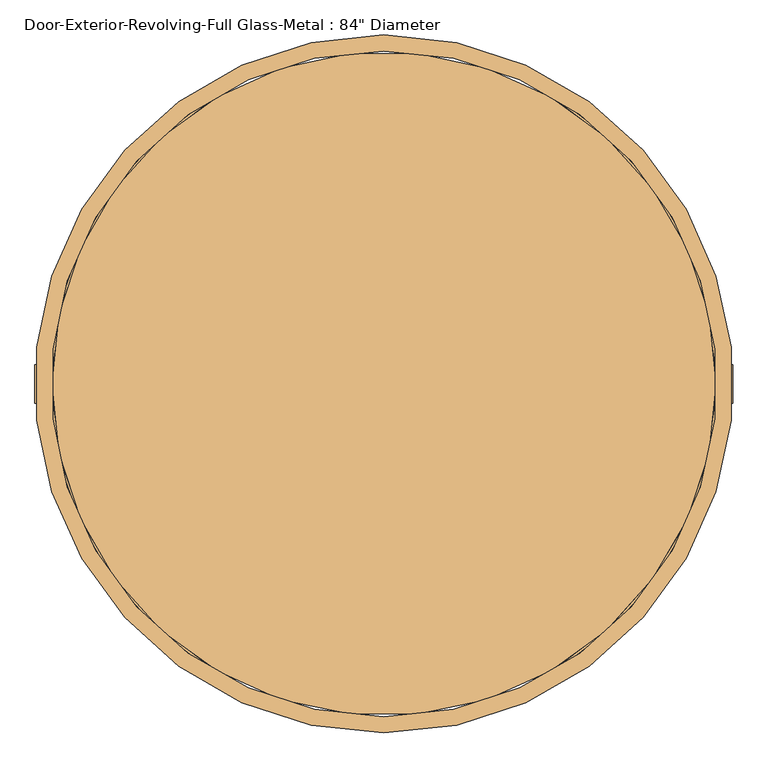
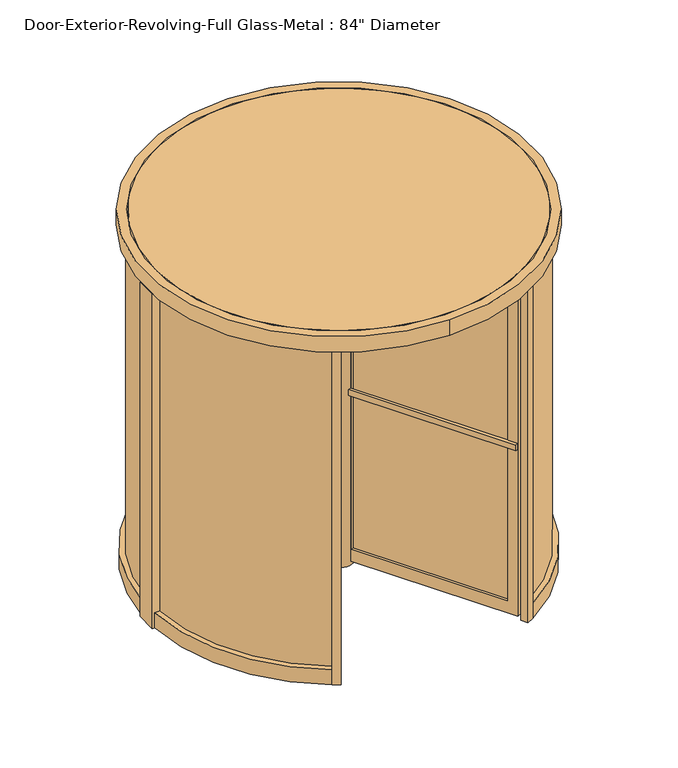
"""IFC4 building model written with IfcOpenShell, lengths in millimetres: door geometry."""

import ifcopenshell
import ifcopenshell.guid

model = None  # the IFC model being written
_history = None  # IfcOwnerHistory: only IFC2X3 demands one
_inside = {}  # id of a spatial element -> (the spatial element, [elements in it])
_under = {}  # id of a project, library or spatial element -> (it, [spatial elements below it])
_declared = {}  # id of a project -> (the project, [libraries it declares])
_typed = {}  # id of a type object -> (the type object, [elements of that type])
_made_of = {}  # id of a material, layer set ... -> (it, [elements and type objects made of it])


def new_model(schema):
    """Start an empty IFC model of exactly this schema.

    Asked for "IFC4X3", IfcOpenShell would pick the latest addendum, in which some entities
    have other attributes; the version numbers below select the first issue.
    IFC2X3 requires an IfcOwnerHistory on every rooted entity: one is made here for all.
    """
    global model, _history
    if schema == "IFC4X3":
        model = ifcopenshell.file(schema_version=(4, 3, 0, 0))
    else:
        model = ifcopenshell.file(schema=schema)
    _inside.clear()
    _under.clear()
    _declared.clear()
    _typed.clear()
    _made_of.clear()
    _history = None
    if model.schema == "IFC2X3":
        org = make("IfcOrganization", Name="unknown")
        user = make(
            "IfcPersonAndOrganization",
            ThePerson=make("IfcPerson", FamilyName="unknown"),
            TheOrganization=org,
        )
        app = make(
            "IfcApplication",
            ApplicationDeveloper=org,
            Version="unknown",
            ApplicationFullName="unknown",
            ApplicationIdentifier="unknown",
        )
        _history = make(
            "IfcOwnerHistory",
            OwningUser=user,
            OwningApplication=app,
            ChangeAction="ADDED",
            CreationDate=0,
        )
    return model


def make(cls, **values):
    """One entity of the class cls with the attributes given. An attribute that is None is left unset."""
    return model.create_entity(
        cls, **{name: value for name, value in values.items() if value is not None}
    )


def rooted(cls, **values):
    """An entity with a GlobalId (a new one), such as an element, a storey or a relation."""
    return make(cls, GlobalId=ifcopenshell.guid.new(), OwnerHistory=_history, **values)


def si_unit(unit_type, name, prefix=None):
    """IfcSIUnit, for example si_unit("LENGTHUNIT", "METRE", prefix="MILLI")."""
    return make("IfcSIUnit", UnitType=unit_type, Prefix=prefix, Name=name)


def assignment(units):
    """IfcUnitAssignment: the units of a project."""
    return None if units is None else make("IfcUnitAssignment", Units=units)


def point(xyz):
    """IfcCartesianPoint."""
    return None if xyz is None else make("IfcCartesianPoint", Coordinates=xyz)


def direction(xyz):
    """IfcDirection."""
    return None if xyz is None else make("IfcDirection", DirectionRatios=xyz)


def frame(location, z_axis=None, x_axis=None):
    """IfcAxis2Placement3D, a coordinate frame: its origin and axes. An axis left out is left unset."""
    return make(
        "IfcAxis2Placement3D",
        Location=point(location),
        Axis=direction(z_axis),
        RefDirection=direction(x_axis),
    )


def frame_2d(location, x_axis=None):
    """IfcAxis2Placement2D, a coordinate frame in the plane: its origin and x axis."""
    return make(
        "IfcAxis2Placement2D", Location=point(location), RefDirection=direction(x_axis)
    )


def origin():
    """The frame at (0, 0, 0) with its axes left unset."""
    return frame((0.0, 0.0, 0.0))


def origin_with_axes():
    """The frame at (0, 0, 0) with the z axis (0, 0, 1) and the x axis (1, 0, 0) written out."""
    return frame((0.0, 0.0, 0.0), z_axis=(0.0, 0.0, 1.0), x_axis=(1.0, 0.0, 0.0))


def origin_2d():
    """The frame at (0, 0) in the plane with its x axis left unset."""
    return frame_2d((0.0, 0.0))


def place(relative_to, where):
    """IfcLocalPlacement: puts the frame where relative to a parent placement (None: the world)."""
    return make(
        "IfcLocalPlacement", PlacementRelTo=relative_to, RelativePlacement=where
    )


def context(
    kind, dimensions, precision=None, world=None, true_north=None, identifier=None
):
    """IfcGeometricRepresentationContext, for example the 3D "Model" context."""
    return make(
        "IfcGeometricRepresentationContext",
        ContextIdentifier=identifier,
        ContextType=kind,
        CoordinateSpaceDimension=dimensions,
        Precision=precision,
        WorldCoordinateSystem=world,
        TrueNorth=true_north,
    )


def project(units=None, contexts=None):
    """IfcProject with its units and contexts."""
    return rooted(
        "IfcProject",
        Name="project",
        RepresentationContexts=contexts,
        UnitsInContext=assignment(units),
    )


def spatial(cls, under=None, at=None, **own):
    """A site, building, storey or space (cls), placed at a placement, below another one or the project."""
    s = rooted(cls, ObjectPlacement=at, **own)
    if under is not None:
        _under.setdefault(under.id(), (under, []))[1].append(s)
    return s


def polyline(points):
    """IfcPolyline through the points."""
    return make("IfcPolyline", Points=[point(p) for p in points])


def circle_curve(where, radius):
    """IfcCircle in the frame where."""
    return make("IfcCircle", Position=where, Radius=radius)


def trimmed(basis, trim1, trim2, sense, master):
    """IfcTrimmedCurve: the piece of a basis curve between two trims."""
    return make(
        "IfcTrimmedCurve",
        BasisCurve=basis,
        Trim1=trim1,
        Trim2=trim2,
        SenseAgreement=sense,
        MasterRepresentation=master,
    )


def segment(curve, same_sense, transition):
    """IfcCompositeCurveSegment."""
    return make(
        "IfcCompositeCurveSegment",
        Transition=transition,
        SameSense=same_sense,
        ParentCurve=curve,
    )


def composite_curve(segments, self_intersect=None):
    """IfcCompositeCurve: segments joined end to end."""
    return make("IfcCompositeCurve", Segments=segments, SelfIntersect=self_intersect)


def outline(outer, holes=None, kind="AREA"):
    """IfcArbitraryClosedProfileDef: a profile drawn as a closed curve; with holes, ...WithVoids."""
    if holes is None:
        return make("IfcArbitraryClosedProfileDef", ProfileType=kind, OuterCurve=outer)
    return make(
        "IfcArbitraryProfileDefWithVoids",
        ProfileType=kind,
        OuterCurve=outer,
        InnerCurves=holes,
    )


def extrude(swept, where, along, depth):
    """IfcExtrudedAreaSolid: the profile swept, set in the frame where, extruded along a direction by depth."""
    return make(
        "IfcExtrudedAreaSolid",
        SweptArea=swept,
        Position=where,
        ExtrudedDirection=direction(along),
        Depth=depth,
    )


def shape(context_of_items, identifier, shape_type, items):
    """IfcShapeRepresentation: the items that make up one representation, for example the "Body"."""
    return make(
        "IfcShapeRepresentation",
        ContextOfItems=context_of_items,
        RepresentationIdentifier=identifier,
        RepresentationType=shape_type,
        Items=items,
    )


def source(mapping_origin, context_of_items, identifier, shape_type, items):
    """IfcRepresentationMap: a shape defined once, which mapped items show again and again."""
    return make(
        "IfcRepresentationMap",
        MappingOrigin=mapping_origin,
        MappedRepresentation=shape(context_of_items, identifier, shape_type, items),
    )


def transform(
    local_origin,
    x_axis=None,
    y_axis=None,
    z_axis=None,
    scale=None,
    scale2=None,
    scale3=None,
    uniform=True,
):
    """IfcCartesianTransformationOperator3D, or its non-uniform kind. x_axis, y_axis, z_axis: its Axis1, 2, 3."""
    if uniform:
        return make(
            "IfcCartesianTransformationOperator3D",
            Axis1=direction(x_axis),
            Axis2=direction(y_axis),
            LocalOrigin=point(local_origin),
            Scale=scale,
            Axis3=direction(z_axis),
        )
    return make(
        "IfcCartesianTransformationOperator3DnonUniform",
        Axis1=direction(x_axis),
        Axis2=direction(y_axis),
        LocalOrigin=point(local_origin),
        Scale=scale,
        Axis3=direction(z_axis),
        Scale2=scale2,
        Scale3=scale3,
    )


def mapped(mapping_source, mapping_target):
    """IfcMappedItem: shows the shape of a source again, moved by a transform."""
    return make(
        "IfcMappedItem", MappingSource=mapping_source, MappingTarget=mapping_target
    )


def made_of(thing, what):
    """Note that an element or type object is made of a material, layer set ...; save() writes the relation."""
    if what is not None:
        _made_of.setdefault(what.id(), (what, []))[1].append(thing)
    return thing


def element(
    cls,
    number,
    at=None,
    inside=None,
    cuts=None,
    type_object=None,
    material=None,
    context=None,
    identifier="Body",
    shape_type=None,
    held_by="IfcProductDefinitionShape",
    body=None,
    shapes=None,
    **own,
):
    """One element of the class cls, such as IfcWall. Its Tag is "e" and its number.

    at: its placement. inside: the storey or other place that contains it. cuts: it is an
    opening in that element (IfcRelVoidsElement). A single representation is given by context,
    identifier, shape_type and body (its items); several are given by shapes. held_by: the class
    of the entity that holds the representations. save() writes the other relations.
    """
    e = rooted(cls, Tag="e%d" % number, ObjectPlacement=at, **own)
    if body is not None:
        shapes = [shape(context, identifier, shape_type, body)]
    if shapes is not None:
        e.Representation = make(held_by, Representations=shapes)
    if inside is not None:
        _inside.setdefault(inside.id(), (inside, []))[1].append(e)
    if cuts is not None:
        rooted(
            "IfcRelVoidsElement", RelatingBuildingElement=cuts, RelatedOpeningElement=e
        )
    if type_object is not None:
        _typed.setdefault(type_object.id(), (type_object, []))[1].append(e)
    return made_of(e, material)


def aggregate(whole, parts):
    """IfcRelAggregates: a whole, such as a stair, and the parts it consists of."""
    return rooted("IfcRelAggregates", RelatingObject=whole, RelatedObjects=parts)


def save(model, path):
    """Write the relations noted so far, then the file.

    IfcRelAggregates (storeys below a building ...), IfcRelContainedInSpatialStructure (elements
    in a storey), IfcRelDefinesByType, IfcRelAssociatesMaterial and IfcRelDeclares: one each for
    every whole, place, type object, material and project.
    """
    for whole, parts in _under.values():
        aggregate(whole, parts)
    for where, things in _inside.values():
        rooted(
            "IfcRelContainedInSpatialStructure",
            RelatedElements=things,
            RelatingStructure=where,
        )
    for kind, things in _typed.values():
        rooted("IfcRelDefinesByType", RelatedObjects=things, RelatingType=kind)
    for what, things in _made_of.values():
        rooted("IfcRelAssociatesMaterial", RelatedObjects=things, RelatingMaterial=what)
    for by, libraries in _declared.values():
        rooted("IfcRelDeclares", RelatingContext=by, RelatedDefinitions=libraries)
    model.write(path)


def plane_surface(at):
    """IfcPlane: the flat surface through the origin of the frame at, square to its z axis."""
    return make("IfcPlane", Position=at)


def revolved_surface(curve, axis_point, axis_direction):
    """IfcSurfaceOfRevolution: the curve turned about the line through axis_point along axis_direction."""
    return make(
        "IfcSurfaceOfRevolution",
        SweptCurve=make("IfcArbitraryOpenProfileDef", ProfileType="CURVE", Curve=curve),
        AxisPosition=make("IfcAxis1Placement", Location=point(axis_point), Axis=direction(axis_direction)),
    )


def advanced_brep(points, edges, surfaces, faces):
    """IfcAdvancedBrep: a solid bounded by faces that lie on surfaces and meet in shared edges.

    An edge is (start, end): straight between two places in points (the first is 0);
    or (start, end, curve); or (start, end, curve, False) where it runs against its curve.
    A face is (place in surfaces, loops), or (place, loops, False) where it looks against
    its surface's normal. A loop lists edges by number (the first is 1), with a minus sign
    where the edge is run from its end to its start. The first loop is the outer one.
    """
    corners = [point(p) for p in points]
    vertices = [make("IfcVertexPoint", VertexGeometry=c) for c in corners]
    made = []
    for start, end, *more in edges:
        made.append(
            make(
                "IfcEdgeCurve",
                EdgeStart=vertices[start],
                EdgeEnd=vertices[end],
                EdgeGeometry=more[0] if more else make("IfcPolyline", Points=[corners[start], corners[end]]),
                SameSense=more[1] if len(more) > 1 else True,
            )
        )
    hull = []
    for where, loops, *sense in faces:
        bounds = []
        for j, loop in enumerate(loops):
            ring = [make("IfcOrientedEdge", EdgeElement=made[abs(k) - 1], Orientation=k > 0) for k in loop]
            bounds.append(
                make(
                    "IfcFaceOuterBound" if j == 0 else "IfcFaceBound",
                    Bound=make("IfcEdgeLoop", EdgeList=ring),
                    Orientation=True,
                )
            )
        hull.append(make("IfcAdvancedFace", Bounds=bounds, FaceSurface=surfaces[where], SameSense=sense[0] if sense else True))
    return make("IfcAdvancedBrep", Outer=make("IfcClosedShell", CfsFaces=hull))


def door_f17faca2(model_context):
    return source(origin(), model_context, "Body", "SolidModel", [
        advanced_brep(
        [(44.45, -76.9896584, 25.4), (44.45, -76.9896584, 2219.325), (59.9152559, -65.6762674, 2219.325), (59.9152559, -65.6762674, 25.4), (26.9196881, -84.7262674, 25.4), (26.9196881, -84.7262674, 2219.325), (558.1772161, -1004.8912978, 25.4), (558.1772161, -1004.8912978, 2219.325), (29.5397161, -89.2642891, 2152.65), (524.8397161, -947.149054, 2152.65), (524.8397161, -947.149054, 106.3625), (29.5397161, -89.2642891, 106.3625), (591.1727839, -985.8412978, 2219.325), (591.1727839, -985.8412978, 25.4), (62.5352839, -70.2142891, 2152.65), (62.5352839, -70.2142891, 106.3625), (557.8352839, -928.099054, 106.3625), (557.8352839, -928.099054, 2152.65)],
        [
            (0, 1),
            (1, 2, circle_curve(frame((0.0, 0.0, 2219.325), z_axis=(0.0, 0.0, 1.0), x_axis=(0.4999999999999996, -0.8660254037844389, 0.0)), 88.9)),
            (2, 3),
            (3, 0, circle_curve(frame((0.0, 0.0, 25.4), z_axis=(0.0, 0.0, -1.0), x_axis=(0.4999999999999996, -0.8660254037844389, 0.0)), 88.9)),
            (0, 4, circle_curve(frame((0.0, 0.0, 25.4), z_axis=(0.0, 0.0, -1.0), x_axis=(0.4999999999999996, -0.8660254037844389, 0.0)), 88.9)),
            (4, 5),
            (5, 1, circle_curve(frame((0.0, 0.0, 2219.325), z_axis=(0.0, 0.0, 1.0), x_axis=(0.4999999999999996, -0.8660254037844389, 0.0)), 88.9)),
            (6, 7),
            (7, 5),
            (4, 6),
            (8, 9),
            (9, 10),
            (10, 11),
            (11, 8),
            (12, 13),
            (13, 3),
            (2, 12),
            (14, 15),
            (15, 16),
            (16, 17),
            (17, 14),
            (7, 12),
            (6, 13),
            (11, 15),
            (14, 8),
            (10, 16),
            (9, 17),
        ],
        [
            revolved_surface(polyline([(44.44999999999997, -76.98965839643662, 2219.325), (44.44999999999997, -76.98965839643662, 25.399999999999977)]), (0.0, 0.0, -344.4385455), (0.0, 0.0, 1.0)),
            plane_surface(frame((-3.7977839, -31.5220453, 2219.325), z_axis=(-0.8660254037844389, -0.4999999999999996, 0.0), x_axis=(0.0, 0.0, -1.0))),
            plane_surface(frame((29.1977839, -12.4720453, 2219.325), z_axis=(0.8660254037844389, 0.4999999999999996, 0.0), x_axis=(0.0, 0.0, 1.0))),
            plane_surface(frame((558.1772161, -1004.8912978, 2219.325), z_axis=(0.0, 0.0, 1.0), x_axis=(0.8660254037844384, 0.5000000000000004, 0.0))),
            plane_surface(frame((558.1772161, -1004.8912978, 25.4), z_axis=(0.5000000000000004, -0.8660254037844384, 0.0), x_axis=(0.8660254037844384, 0.5000000000000004, 0.0))),
            plane_surface(frame((-3.7977839, -31.5220453, 25.4), z_axis=(0.0, 0.0, -1.0), x_axis=(0.8660254037844389, 0.49999999999999956, 0.0))),
            plane_surface(frame((29.5397161, -89.2642891, 106.3625), z_axis=(0.49999999999999983, -0.8660254037844388, 0.0), x_axis=(0.8660254037844388, 0.49999999999999983, 0.0))),
            plane_surface(frame((524.8397161, -947.149054, 106.3625), z_axis=(0.0, 0.0, 1.0), x_axis=(0.8660254037844404, 0.49999999999999706, 0.0))),
            plane_surface(frame((524.8397161, -947.149054, 2152.65), z_axis=(-0.49999999999999706, 0.8660254037844404, 0.0), x_axis=(0.8660254037844404, 0.49999999999999706, 0.0))),
            plane_surface(frame((29.5397161, -89.2642891, 2152.65), z_axis=(0.0, 0.0, -1.0), x_axis=(0.8660254037844389, 0.49999999999999967, 0.0))),
        ],
        [
            (0, [[1, 2, 3, 4]]),
            (0, [[-1, 5, 6, 7]]),
            (1, [[8, 9, -6, 10], [11, 12, 13, 14]]),
            (2, [[15, 16, -3, 17], [18, 19, 20, 21]]),
            (3, [[22, -17, -2, -7, -9]]),
            (4, [[-8, 23, -15, -22]]),
            (5, [[-23, -10, -5, -4, -16]]),
            (6, [[-14, 24, -18, 25]]),
            (7, [[-13, 26, -19, -24]]),
            (8, [[-12, 27, -20, -26]]),
            (9, [[-11, -25, -21, -27]]),
        ],
    ),
        advanced_brep(
        [(-1149.35, -19.05, 2219.325), (-1149.35, -19.05, 25.4), (-86.834944, -19.05, 25.4), (-86.834944, -19.05, 2219.325), (-92.075, -19.05, 2152.65), (-92.075, -19.05, 106.3625), (-1082.675, -19.05, 106.3625), (-1082.675, -19.05, 2152.65), (-1149.35, 19.05, 25.4), (-1149.35, 19.05, 2219.325), (-86.834944, 19.05, 2219.325), (-86.834944, 19.05, 25.4), (-92.075, 19.05, 2152.65), (-1082.675, 19.05, 2152.65), (-1082.675, 19.05, 106.3625), (-92.075, 19.05, 106.3625)],
        [
            (0, 1),
            (1, 2),
            (2, 3),
            (3, 0),
            (4, 5),
            (5, 6),
            (6, 7),
            (7, 4),
            (8, 9),
            (9, 10),
            (10, 11),
            (11, 8),
            (12, 13),
            (13, 14),
            (14, 15),
            (15, 12),
            (9, 0),
            (3, 10, circle_curve(frame((0.0, 0.0, 2219.325), z_axis=(0.0, 0.0, -1.0), x_axis=(0.4999999999999996, -0.8660254037844389, 0.0)), 88.9)),
            (8, 1),
            (11, 2, circle_curve(frame((0.0, 0.0, 25.4), z_axis=(0.0, 0.0, 1.0), x_axis=(0.4999999999999996, -0.8660254037844389, 0.0)), 88.9)),
            (4, 12),
            (15, 5),
            (14, 6),
            (13, 7),
        ],
        [
            plane_surface(frame((-1149.35, -19.05, 2219.325), z_axis=(0.0, -1.0, 0.0), x_axis=(-1.0, 0.0, 0.0))),
            plane_surface(frame((-1149.35, 19.05, 2219.325), z_axis=(0.0, 1.0, 0.0), x_axis=(1.0, 0.0, 0.0))),
            plane_surface(frame((-25.4, -19.05, 2219.325), z_axis=(0.0, 0.0, 1.0), x_axis=(0.0, 1.0, 0.0))),
            plane_surface(frame((-1149.35, -19.05, 2219.325), z_axis=(-1.0, 0.0, 0.0), x_axis=(0.0, 1.0, 0.0))),
            plane_surface(frame((-1149.35, -19.05, 25.4), z_axis=(0.0, 0.0, -1.0), x_axis=(0.0, 1.0, 0.0))),
            plane_surface(frame((-92.075, -19.05, 2152.65), z_axis=(-1.0, 0.0, 0.0), x_axis=(0.0, 1.0, 0.0))),
            plane_surface(frame((-92.075, -19.05, 106.3625), z_axis=(0.0, 0.0, 1.0), x_axis=(0.0, 1.0, 0.0))),
            plane_surface(frame((-1082.675, -19.05, 106.3625), z_axis=(1.0, 0.0, 0.0), x_axis=(0.0, 1.0, 0.0))),
            plane_surface(frame((-1082.675, -19.05, 2152.65), z_axis=(0.0, 0.0, -1.0), x_axis=(0.0, 1.0, 0.0))),
            revolved_surface(polyline([(44.44999999999997, -76.98965839643662, 2219.325), (44.44999999999997, -76.98965839643662, 25.399999999999977)]), (0.0, 0.0, -344.4385455), (0.0, 0.0, 1.0)),
        ],
        [
            (0, [[1, 2, 3, 4], [5, 6, 7, 8]]),
            (1, [[9, 10, 11, 12], [13, 14, 15, 16]]),
            (2, [[17, -4, 18, -10]]),
            (3, [[-1, -17, -9, 19]]),
            (4, [[-19, -12, 20, -2]]),
            (5, [[-5, 21, -16, 22]]),
            (6, [[-6, -22, -15, 23]]),
            (7, [[-7, -23, -14, 24]]),
            (8, [[-8, -24, -13, -21]]),
            (9, [[-3, -20, -11, -18]]),
        ],
    ),
        advanced_brep(
        [(591.1727839, 985.8412978, 25.4), (591.1727839, 985.8412978, 2219.325), (59.9152559, 65.6762674, 2219.325), (59.9152559, 65.6762674, 25.4), (62.5352839, 70.2142891, 2152.65), (557.8352839, 928.099054, 2152.65), (557.8352839, 928.099054, 106.3625), (62.5352839, 70.2142891, 106.3625), (558.1772161, 1004.8912978, 2219.325), (558.1772161, 1004.8912978, 25.4), (26.9196881, 84.7262674, 25.4), (26.9196881, 84.7262674, 2219.325), (29.5397161, 89.2642891, 2152.65), (29.5397161, 89.2642891, 106.3625), (524.8397161, 947.149054, 106.3625), (524.8397161, 947.149054, 2152.65)],
        [
            (0, 1),
            (1, 2),
            (2, 3),
            (3, 0),
            (4, 5),
            (5, 6),
            (6, 7),
            (7, 4),
            (8, 9),
            (9, 10),
            (10, 11),
            (11, 8),
            (12, 13),
            (13, 14),
            (14, 15),
            (15, 12),
            (1, 8),
            (11, 2, circle_curve(frame((0.0, 0.0, 2219.325), z_axis=(0.0, 0.0, -1.0), x_axis=(0.4999999999999996, -0.8660254037844389, 0.0)), 88.9)),
            (0, 9),
            (3, 10, circle_curve(frame((0.0, 0.0, 25.4), z_axis=(0.0, 0.0, 1.0), x_axis=(0.4999999999999996, -0.8660254037844389, 0.0)), 88.9)),
            (7, 13),
            (12, 4),
            (6, 14),
            (5, 15),
        ],
        [
            plane_surface(frame((29.1977839, 12.4720453, 2219.325), z_axis=(0.866025403784439, -0.4999999999999995, 0.0), x_axis=(0.0, 0.0, -1.0))),
            plane_surface(frame((-3.7977839, 31.5220453, 2219.325), z_axis=(-0.866025403784439, 0.4999999999999995, 0.0), x_axis=(0.0, 0.0, 1.0))),
            plane_surface(frame((591.1727839, 985.8412978, 2219.325), z_axis=(0.0, 0.0, 1.0), x_axis=(-0.8660254037844384, 0.5000000000000004, 0.0))),
            plane_surface(frame((591.1727839, 985.8412978, 25.4), z_axis=(0.5000000000000004, 0.8660254037844384, 0.0), x_axis=(-0.8660254037844384, 0.5000000000000004, 0.0))),
            plane_surface(frame((29.1977839, 12.4720453, 25.4), z_axis=(0.0, 0.0, -1.0), x_axis=(-0.866025403784439, 0.49999999999999944, 0.0))),
            plane_surface(frame((62.5352839, 70.2142891, 106.3625), z_axis=(0.49999999999999967, 0.8660254037844388, 0.0), x_axis=(-0.8660254037844388, 0.49999999999999967, 0.0))),
            plane_surface(frame((557.8352839, 928.099054, 106.3625), z_axis=(0.0, 0.0, 1.0), x_axis=(-0.8660254037844384, 0.5000000000000004, 0.0))),
            plane_surface(frame((557.8352839, 928.099054, 2152.65), z_axis=(-0.5000000000000004, -0.8660254037844384, 0.0), x_axis=(-0.8660254037844384, 0.5000000000000004, 0.0))),
            plane_surface(frame((62.5352839, 70.2142891, 2152.65), z_axis=(0.0, 0.0, -1.0), x_axis=(-0.866025403784439, 0.49999999999999944, 0.0))),
            revolved_surface(polyline([(44.44999999999997, -76.98965839643662, 2219.325), (44.44999999999997, -76.98965839643662, 25.399999999999977)]), (0.0, 0.0, -344.4385455), (0.0, 0.0, 1.0)),
        ],
        [
            (0, [[1, 2, 3, 4], [5, 6, 7, 8]]),
            (1, [[9, 10, 11, 12], [13, 14, 15, 16]]),
            (2, [[17, -12, 18, -2]]),
            (3, [[-1, 19, -9, -17]]),
            (4, [[-19, -4, 20, -10]]),
            (5, [[-8, 21, -13, 22]]),
            (6, [[-7, 23, -14, -21]]),
            (7, [[-6, 24, -15, -23]]),
            (8, [[-5, -22, -16, -24]]),
            (9, [[-3, -18, -11, -20]]),
        ],
    ),
        extrude(outline(composite_curve([segment(polyline([(-615.7921907, 989.2164973), (-638.1275667, 1031.4059972)]), True, "CONTINUOUS"), segment(trimmed(circle_curve(origin_2d(), 1212.85), [point((-638.1275667, 1031.4059972))], [point((-595.6078601, 1056.530359))], False, "CARTESIAN"), True, "CONTINUOUS"), segment(polyline([(-595.6078601, 1056.530359), (-573.2795251, 1014.4456056)]), True, "CONTINUOUS"), segment(trimmed(circle_curve(origin_2d(), 1165.225), [point((-573.2795251, 1014.4456056))], [point((-615.7921907, 989.2164973))], True, "CARTESIAN"), True, "CONTINUOUS")], self_intersect=False)), origin_with_axes(), (0.0, 0.0, 1.0), 2244.725),
        extrude(outline(composite_curve([segment(polyline([(638.2334006, 1031.6059079), (615.7921907, 989.2164973)]), True, "CONTINUOUS"), segment(trimmed(circle_curve(origin_2d(), 1165.225), [point((615.7921907, 989.2164973))], [point((573.2795251, 1014.4456056))], True, "CARTESIAN"), True, "CONTINUOUS"), segment(polyline([(573.2795251, 1014.4456056), (595.7136707, 1056.7297882)]), True, "CONTINUOUS"), segment(trimmed(circle_curve(origin_2d(), 1213.0756872), [point((595.7136707, 1056.7297882))], [point((638.2334006, 1031.6059079))], False, "CARTESIAN"), True, "CONTINUOUS")], self_intersect=False)), origin_with_axes(), (0.0, 0.0, 1.0), 2244.725),
        extrude(outline(composite_curve([segment(trimmed(circle_curve(origin_2d(), 1165.225), [point((-615.7921907, -989.2164973))], [point((-573.2795251, -1014.4456056))], True, "CARTESIAN"), True, "CONTINUOUS"), segment(polyline([(-573.2795251, -1014.4456056), (-595.6078601, -1052.8850325)]), True, "CONTINUOUS"), segment(trimmed(circle_curve(frame_2d((0.0, 179.0003095)), 1368.3165638), [point((-595.6078601, -1052.8850325))], [point((-638.1275667, -1031.4059972))], False, "CARTESIAN"), True, "CONTINUOUS"), segment(polyline([(-638.1275667, -1031.4059972), (-615.7921907, -989.2164973)]), True, "CONTINUOUS")], self_intersect=False)), origin_with_axes(), (0.0, 0.0, 1.0), 2244.725),
        extrude(outline(composite_curve([segment(trimmed(circle_curve(frame_2d((0.0, 179.0003498)), 1368.3165995), [point((638.1275667, -1031.4059972))], [point((595.6078689, -1052.8850275))], False, "CARTESIAN"), True, "CONTINUOUS"), segment(polyline([(595.6078689, -1052.8850275), (573.2795251, -1014.4456056)]), True, "CONTINUOUS"), segment(trimmed(circle_curve(origin_2d(), 1165.225), [point((573.2795251, -1014.4456056))], [point((615.7921907, -989.2164973))], True, "CARTESIAN"), True, "CONTINUOUS"), segment(polyline([(615.7921907, -989.2164973), (638.1275667, -1031.4059972)]), True, "CONTINUOUS")], self_intersect=False)), origin_with_axes(), (0.0, 0.0, 1.0), 2244.725),
        extrude(outline(composite_curve([segment(polyline([(-1171.2208243, 67.46875), (-1177.5812382, 67.46875)]), True, "CONTINUOUS"), segment(trimmed(circle_curve(origin_2d(), 1179.5124437), [point((-1177.5812382, 67.46875))], [point((-622.9714922, 1001.5768191))], False, "CARTESIAN"), True, "CONTINUOUS"), segment(polyline([(-622.9714922, 1001.5768191), (-619.7807004, 996.0833975)]), True, "CONTINUOUS"), segment(trimmed(circle_curve(origin_2d(), 1173.1625), [point((-619.7807004, 996.0833975))], [point((-1171.2208243, 67.46875))], True, "CARTESIAN"), True, "CONTINUOUS")], self_intersect=False)), frame((0.0, 0.0, 101.6), z_axis=(0.0, 0.0, 1.0), x_axis=(1.0, 0.0, 0.0)), (0.0, 0.0, 1.0), 2143.125),
        extrude(outline(composite_curve([segment(trimmed(circle_curve(origin_2d(), 1173.1625), [point((1171.2208243, 67.46875))], [point((619.7807004, 996.0833975))], True, "CARTESIAN"), True, "CONTINUOUS"), segment(polyline([(619.7807004, 996.0833975), (622.9714922, 1001.5768191)]), True, "CONTINUOUS"), segment(trimmed(circle_curve(origin_2d(), 1179.5124437), [point((622.9714922, 1001.5768191))], [point((1177.5812382, 67.46875))], False, "CARTESIAN"), True, "CONTINUOUS"), segment(polyline([(1177.5812382, 67.46875), (1171.2208243, 67.46875)]), True, "CONTINUOUS")], self_intersect=False)), frame((0.0, 0.0, 101.6), z_axis=(0.0, 0.0, 1.0), x_axis=(1.0, 0.0, 0.0)), (0.0, 0.0, 1.0), 2143.125),
        extrude(outline(composite_curve([segment(trimmed(circle_curve(origin_2d(), 1173.1625), [point((-1171.2208243, -67.46875))], [point((-619.7807004, -996.0833975))], True, "CARTESIAN"), True, "CONTINUOUS"), segment(polyline([(-619.7807004, -996.0833975), (-622.9714922, -1001.5768191)]), True, "CONTINUOUS"), segment(trimmed(circle_curve(origin_2d(), 1179.5124437), [point((-622.9714922, -1001.5768191))], [point((-1177.5812382, -67.46875))], False, "CARTESIAN"), True, "CONTINUOUS"), segment(polyline([(-1177.5812382, -67.46875), (-1171.2208243, -67.46875)]), True, "CONTINUOUS")], self_intersect=False)), frame((0.0, 0.0, 101.6), z_axis=(0.0, 0.0, 1.0), x_axis=(1.0, 0.0, 0.0)), (0.0, 0.0, 1.0), 2143.125),
        extrude(outline(composite_curve([segment(polyline([(1171.2208243, -67.46875), (1177.5812382, -67.46875)]), True, "CONTINUOUS"), segment(trimmed(circle_curve(origin_2d(), 1179.5124437), [point((1177.5812382, -67.46875))], [point((622.9714922, -1001.5768191))], False, "CARTESIAN"), True, "CONTINUOUS"), segment(polyline([(622.9714922, -1001.5768191), (619.7807004, -996.0833975)]), True, "CONTINUOUS"), segment(trimmed(circle_curve(origin_2d(), 1173.1625), [point((619.7807004, -996.0833975))], [point((1171.2208243, -67.46875))], True, "CARTESIAN"), True, "CONTINUOUS")], self_intersect=False)), frame((0.0, 0.0, 101.6), z_axis=(0.0, 0.0, 1.0), x_axis=(1.0, 0.0, 0.0)), (0.0, 0.0, 1.0), 2143.125),
        extrude(outline(composite_curve([segment(trimmed(circle_curve(origin_2d(), 1225.55), [point((0.0, -1225.55))], [point((0.0, 1225.55))], False, "CARTESIAN"), True, "CONTINUOUS"), segment(trimmed(circle_curve(origin_2d(), 1225.55), [point((0.0, 1225.55))], [point((0.0, -1225.55))], False, "CARTESIAN"), True, "CONTINUOUS")], self_intersect=False), holes=[composite_curve([segment(trimmed(circle_curve(origin_2d(), 1168.4), [point((0.0, 1168.4))], [point((0.0, -1168.4))], True, "CARTESIAN"), True, "CONTINUOUS"), segment(trimmed(circle_curve(origin_2d(), 1168.4), [point((0.0, -1168.4))], [point((0.0, 1168.4))], True, "CARTESIAN"), True, "CONTINUOUS")], self_intersect=False)]), frame((0.0, 0.0, 2244.725), z_axis=(0.0, 0.0, 1.0), x_axis=(1.0, 0.0, 0.0)), (0.0, 0.0, 1.0), 101.6),
        extrude(outline(composite_curve([segment(trimmed(circle_curve(origin_2d(), 1165.225), [point((-1165.225, 0.0))], [point((1165.225, 0.0))], False, "CARTESIAN"), True, "CONTINUOUS"), segment(trimmed(circle_curve(origin_2d(), 1165.225), [point((1165.225, 0.0))], [point((-1165.225, 0.0))], False, "CARTESIAN"), True, "CONTINUOUS")], self_intersect=False)), frame((0.0, 0.0, 2244.725), z_axis=(0.0, 0.0, 1.0), x_axis=(1.0, 0.0, 0.0)), (0.0, 0.0, 1.0), 101.6),
        extrude(outline(composite_curve([segment(trimmed(circle_curve(origin_2d(), 88.9), [point((-88.9, 0.0))], [point((88.9, 0.0))], False, "CARTESIAN"), True, "CONTINUOUS"), segment(trimmed(circle_curve(origin_2d(), 88.9), [point((88.9, 0.0))], [point((-88.9, 0.0))], False, "CARTESIAN"), True, "CONTINUOUS")], self_intersect=False)), origin_with_axes(), (0.0, 0.0, 1.0), 2244.725),
        extrude(outline(composite_curve([segment(polyline([(-615.7921907, -989.2164973), (-638.1275667, -1031.4059972)]), True, "CONTINUOUS"), segment(trimmed(circle_curve(origin_2d(), 1212.85), [point((-638.1275667, -1031.4059972))], [point((-1210.971961, -67.46875))], False, "CARTESIAN"), True, "CONTINUOUS"), segment(polyline([(-1210.971961, -67.46875), (-1163.2700754, -67.46875)]), True, "CONTINUOUS"), segment(trimmed(circle_curve(origin_2d(), 1165.225), [point((-1163.2700754, -67.46875))], [point((-615.7921907, -989.2164973))], True, "CARTESIAN"), True, "CONTINUOUS")], self_intersect=False)), origin_with_axes(), (0.0, 0.0, 1.0), 101.6),
        extrude(outline(composite_curve([segment(polyline([(638.1275667, -1031.4059972), (615.7921907, -989.2164973)]), True, "CONTINUOUS"), segment(trimmed(circle_curve(origin_2d(), 1165.225), [point((615.7921907, -989.2164973))], [point((1163.2700754, -67.46875))], True, "CARTESIAN"), True, "CONTINUOUS"), segment(polyline([(1163.2700754, -67.46875), (1210.971961, -67.46875)]), True, "CONTINUOUS"), segment(trimmed(circle_curve(origin_2d(), 1212.85), [point((1210.971961, -67.46875))], [point((638.1275667, -1031.4059972))], False, "CARTESIAN"), True, "CONTINUOUS")], self_intersect=False)), origin_with_axes(), (0.0, 0.0, 1.0), 101.6),
        extrude(outline(composite_curve([segment(polyline([(1210.971961, 67.46875), (1163.2700754, 67.46875)]), True, "CONTINUOUS"), segment(trimmed(circle_curve(origin_2d(), 1165.225), [point((1163.2700754, 67.46875))], [point((615.7921907, 989.2164973))], True, "CARTESIAN"), True, "CONTINUOUS"), segment(polyline([(615.7921907, 989.2164973), (638.1275667, 1031.4059972)]), True, "CONTINUOUS"), segment(trimmed(circle_curve(origin_2d(), 1212.85), [point((638.1275667, 1031.4059972))], [point((1210.971961, 67.46875))], False, "CARTESIAN"), True, "CONTINUOUS")], self_intersect=False)), origin_with_axes(), (0.0, 0.0, 1.0), 101.6),
        extrude(outline(composite_curve([segment(polyline([(-638.1275667, 1031.4059972), (-615.7921907, 989.2164973)]), True, "CONTINUOUS"), segment(trimmed(circle_curve(origin_2d(), 1165.225), [point((-615.7921907, 989.2164973))], [point((-1163.2700754, 67.46875))], True, "CARTESIAN"), True, "CONTINUOUS"), segment(polyline([(-1163.2700754, 67.46875), (-1210.971961, 67.46875)]), True, "CONTINUOUS"), segment(trimmed(circle_curve(origin_2d(), 1212.85), [point((-1210.971961, 67.46875))], [point((-638.1275667, 1031.4059972))], False, "CARTESIAN"), True, "CONTINUOUS")], self_intersect=False)), origin_with_axes(), (0.0, 0.0, 1.0), 101.6),
        extrude(outline(polyline([(-1168.4, 67.46875), (-1168.4, -67.46875), (-1225.55, -67.46875), (-1225.55, 67.46875), (-1168.4, 67.46875)])), origin_with_axes(), (0.0, 0.0, 1.0), 2244.725),
        extrude(outline(polyline([(1225.55, 67.46875), (1225.55, -67.46875), (1168.4, -67.46875), (1168.4, 67.46875), (1225.55, 67.46875)])), origin_with_axes(), (0.0, 0.0, 1.0), 2244.725),
        extrude(outline(polyline([(538.5878693, -939.211554), (43.2878693, -81.3267891), (48.7871307, -78.1517891), (544.0871307, -936.036554), (538.5878693, -939.211554)])), frame((0.0, 0.0, 106.3625), z_axis=(0.0, 0.0, 1.0), x_axis=(1.0, 0.0, 0.0)), (0.0, 0.0, 1.0), 2046.2875),
        extrude(outline(polyline([(544.0871307, 936.036554), (48.7871307, 78.1517891), (43.2878693, 81.3267891), (538.5878693, 939.211554), (544.0871307, 936.036554)])), frame((0.0, 0.0, 106.3625), z_axis=(0.0, 0.0, 1.0), x_axis=(1.0, 0.0, 0.0)), (0.0, 0.0, 1.0), 2046.2875),
        extrude(outline(polyline([(-92.075, -3.175), (-1082.675, -3.175), (-1082.675, 3.175), (-92.075, 3.175), (-92.075, -3.175)])), frame((0.0, 0.0, 106.3625), z_axis=(0.0, 0.0, 1.0), x_axis=(1.0, 0.0, 0.0)), (0.0, 0.0, 1.0), 2046.2875),
        extrude(outline(composite_curve([segment(polyline([(-1149.35, 19.05), (-1149.35, 38.1), (-80.3218526, 38.1)]), True, "CONTINUOUS"), segment(trimmed(circle_curve(origin_2d(), 88.9), [point((-80.3218526, 38.1))], [point((-86.834944, 19.05))], True, "CARTESIAN"), True, "CONTINUOUS"), segment(polyline([(-86.834944, 19.05), (-1149.35, 19.05)]), True, "CONTINUOUS")], self_intersect=False)), frame((0.0, 0.0, 1149.35), z_axis=(0.0, 0.0, 1.0), x_axis=(1.0, 0.0, 0.0)), (0.0, 0.0, 1.0), 38.1),
        extrude(outline(composite_curve([segment(polyline([(558.1772161, -1004.8912978), (541.6794321, -1014.4162978), (7.1653584, -88.6107648)]), True, "CONTINUOUS"), segment(trimmed(circle_curve(origin_2d(), 88.9), [point((7.1653584, -88.6107648))], [point((26.9196881, -84.7262674))], True, "CARTESIAN"), True, "CONTINUOUS"), segment(polyline([(26.9196881, -84.7262674), (558.1772161, -1004.8912978)]), True, "CONTINUOUS")], self_intersect=False)), frame((0.0, 0.0, 1149.35), z_axis=(0.0, 0.0, 1.0), x_axis=(1.0, 0.0, 0.0)), (0.0, 0.0, 1.0), 38.1),
        extrude(outline(composite_curve([segment(polyline([(591.1727839, 985.8412978), (607.6705679, 976.3162978), (73.1564942, 50.5107648)]), True, "CONTINUOUS"), segment(trimmed(circle_curve(origin_2d(), 88.9), [point((73.1564942, 50.5107648))], [point((59.9152559, 65.6762674))], True, "CARTESIAN"), True, "CONTINUOUS"), segment(polyline([(59.9152559, 65.6762674), (591.1727839, 985.8412978)]), True, "CONTINUOUS")], self_intersect=False)), frame((0.0, 0.0, 1149.35), z_axis=(0.0, 0.0, 1.0), x_axis=(1.0, 0.0, 0.0)), (0.0, 0.0, 1.0), 38.1),
    ])


if __name__ == "__main__":
    model = new_model("IFC4")
    model_context = context("Model", 3, world=origin())
    ifc_project = project(units=[si_unit("LENGTHUNIT", "METRE", prefix="MILLI")], contexts=[model_context])
    site = spatial("IfcSite", under=ifc_project)
    building = spatial("IfcBuilding", under=site)
    placement = place(None, origin())
    door_shape = door_f17faca2(model_context)
    element("IfcDoor", 1, ObjectType="Door-Exterior-Revolving-Full Glass-Metal : 84\" Diameter", at=placement, inside=building, context=model_context, shape_type="MappedRepresentation", body=[
        mapped(door_shape, transform((0.0, 0.0, 0.0), x_axis=(1.0, 0.0, 0.0), y_axis=(0.0, 1.0, 0.0), z_axis=(0.0, 0.0, 1.0))),
    ])
    save(model, "model.ifc")

# Revit data of these elements
# Type "Door-Exterior-Revolving-Full Glass-Metal : 84\" Diameter"
#   Type Mark = "35"
#   Assembly Code = "B2030300"
#   Analytic Construction = "Metal frame, double glass door"
#   Width = 8' - 0"
#   Thermal Resistance (R) = 1.3794 (h·ft²·°F)/BTU
#   Rough Width = 8' - 0 1/2"
#   Rough Height = 7' - 8 3/8"
#   Push Bar Height = 3' - 10"
#   Panel Width = 3' - 8 1/4"
#   Outside Diameter = 8' - 0 1/2"
#   Inside Radius = 3' - 9 7/8"
#   Inside Diameter = 7' - 7 3/4"
#   Height = 7' - 8"
#   Heat Transfer Coefficient (U) = 0.7250 BTU/(h·ft²·°F)
#   Glazing Radius = 3' - 10 3/16"
#   Door Opening Width = 3' - 9 1/8"
#   Function = 1
#   Push Bar Material = Aluminum
#   Panel Material = Aluminum
#   Glazing = Glass
#   Frame Material = Aluminum
#   Wall Closure = (empty or 0)
#   Visual Light Transmittance = 0
#   Solar Heat Gain Coefficient = 0
# Element 1 (IfcDoor, "Door-Exterior-Revolving-Full Glass-Metal : 84\" Diameter")
#   Materials on its faces: "Aluminum", "Glass"
# Materials
#   "Aluminum": class "Metal", colour RGB 120 120 120, transparency 0, Description = "Aluminum 6061", Cost = 0
#   "Glass": class "Unassigned", colour RGB 0 128 192, transparency 0.75, Description = "Glass"
